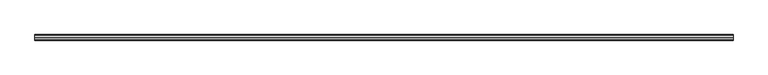
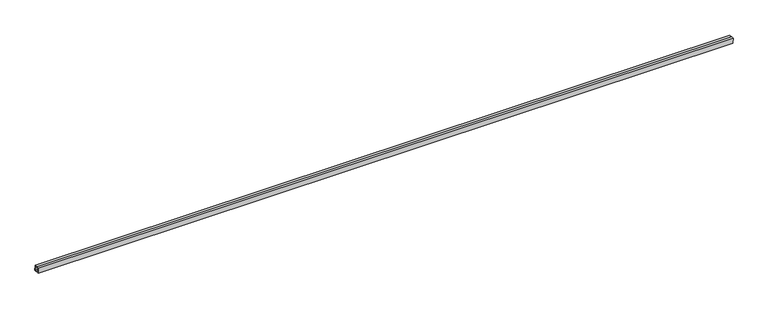
"""IFC4 building model written with IfcOpenShell, lengths in millimetres: proxy geometry, Inner panel:Inner panel:1:Inner panel:1 : Inner panel:Inner panel:300324:2:Inner panel:1:Inner panel:1 : Inner panel:Inner panel:300324:2 : Inner panel:Inner panel:1:Inner panel:1 : Inner panel:Inner panel:300324:300043:56 : Inner panel:Inner panel:1:Inner panel:1 : Inner panel:Inner panel:300324:2:Inner panel:1:Inner panel:1 : Inner panel:Inner panel:300324:2 : Inner panel:Inner panel:1:Inner panel:1 : Inner panel:Inner panel:300324:300043:308120."""

from ifc_helpers import new_model, si_unit, frame, origin, place, context, project, spatial, polyline, outline, extrude, source, transform, mapped, element, save


def generic_models_0f87fd24(model_context):
    return source(origin(), model_context, "Body", "SweptSolid", [
        extrude(outline(polyline([(-577258.3887241, 4022.4942957), (-577240.148301, 4023.2543133), (-577238.5621772, 3985.1873432), (-577276.6291473, 3983.6012194), (-577278.215271, 4021.6681895), (-577259.9748479, 4022.4282072), (-577259.8757151, 4020.0490215), (-577275.7369527, 4019.3881366), (-577274.3490944, 3986.0795378), (-577241.0404956, 3987.4673961), (-577242.4283539, 4020.7759949), (-577258.2895914, 4020.11511), (-577258.3887241, 4022.4942957)])), frame((659327.2367238, 0.0, 0.0), z_axis=(1.0, 0.0, 0.0), x_axis=(0.0, 1.0, 0.0)), (0.0, 0.0, 1.0), 4876.8),
    ])


if __name__ == "__main__":
    model = new_model("IFC4")
    model_context = context("Model", 3, world=origin())
    ifc_project = project(units=[si_unit("LENGTHUNIT", "METRE", prefix="MILLI")], contexts=[model_context])
    site = spatial("IfcSite", under=ifc_project)
    building = spatial("IfcBuilding", under=site)
    placement = place(None, origin())
    generic_models_shape = generic_models_0f87fd24(model_context)
    element("IfcBuildingElementProxy", 1, Name="Inner panel:Inner panel:1:Inner panel:1 : Inner panel:Inner panel:300324:2:Inner panel:1:Inner panel:1 : Inner panel:Inner panel:300324:2 : Inner panel:Inner panel:1:Inner panel:1 : Inner panel:Inner panel:300324:300043:56 : Inner panel:Inner panel:1:Inner panel:1 : Inner panel:Inner panel:300324:2:Inner panel:1:Inner panel:1 : Inner panel:Inner panel:300324:2 : Inner panel:Inner panel:1:Inner panel:1 : Inner panel:Inner panel:300324:300043:308120", ObjectType="Inner panel:Inner panel:1:Inner panel:1 : Inner panel:Inner panel:300324:2:Inner panel:1:Inner panel:1 : Inner panel:Inner panel:300324:2 : Inner panel:Inner panel:1:Inner panel:1 : Inner panel:Inner panel:300324:300043:56 : Inner panel:Inner panel:1:Inner panel:1 : Inner panel:Inner panel:300324:2:Inner panel:1:Inner panel:1 : Inner panel:Inner panel:300324:2 : Inner panel:Inner panel:1:Inner panel:1 : Inner panel:Inner panel:300324:300043:308120", at=placement, inside=building, context=model_context, shape_type="MappedRepresentation", body=[
        mapped(generic_models_shape, transform((0.0, 0.0, 0.0), x_axis=(1.0, 0.0, 0.0), y_axis=(0.0, 1.0, 0.0), z_axis=(0.0, 0.0, 1.0))),
    ])
    save(model, "model.ifc")

# Revit data of these elements
# Type "Inner panel:Inner panel:1:Inner panel:1 : Inner panel:Inner panel:300324:2:Inner panel:1:Inner panel:1 : Inner panel:Inner panel:300324:2 : Inner panel:Inner panel:1:Inner panel:1 : Inner panel:Inner panel:300324:300043:56 : Inner panel:Inner panel:1:Inner panel:1 : Inner panel:Inner panel:300324:2:Inner panel:1:Inner panel:1 : Inner panel:Inner panel:300324:2 : Inner panel:Inner panel:1:Inner panel:1 : Inner panel:Inner panel:300324:300043:308120"
#   NameOverride = "Inner panel:Inner panel:1:Inner panel:1 : Inner panel:Inner panel:300324:2:Inner panel:1:Inner panel:1 : Inner panel:Inner panel:300324:2 : Inner panel:Inner panel:1:Inner panel:1 : Inner panel:Inner panel:300324:300043:308120"
#   ObjectTypeOverride = "Inner panel:1:Inner panel:1 : Inner panel:Inner panel:300324:2 : Inner panel:Inner panel:1:Inner panel:1 : Inner panel:Inner panel:300324:300043"
#   Reference = "Inner panel"
#   Tag = "308120"
# Element 1 (IfcBuildingElementProxy, "Inner panel:Inner panel:1:Inner panel:1 : Inner panel:Inner panel:300324:2:Inner panel:1:Inner panel:1 : Inner panel:Inner panel:300324:2 : Inner panel:Inner panel:1:Inner panel:1 : Inner panel:Inner panel:300324:300043:56 : Inner panel:Inner panel:1:Inner panel:1 : Inner panel:Inner panel:300324:2:Inner panel:1:Inner panel:1 : Inner panel:Inner panel:300324:2 : Inner panel:Inner panel:1:Inner panel:1 : Inner panel:Inner panel:300324:300043:308120")
#   Materials on its faces: "1 1/2\" X 1 1/2\" SPLIT-SEAM SQUARE TUBING (~24\" CANTILEVER FROM C.L. OF GLULAM)"
# Materials
#   "1 1/2\" X 1 1/2\" SPLIT-SEAM SQUARE TUBING (~24\" CANTILEVER FROM C.L. OF GLULAM)": class "Unassigned", colour RGB 202 201 200, transparency 0, Cost = 0
